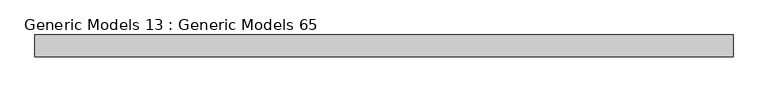
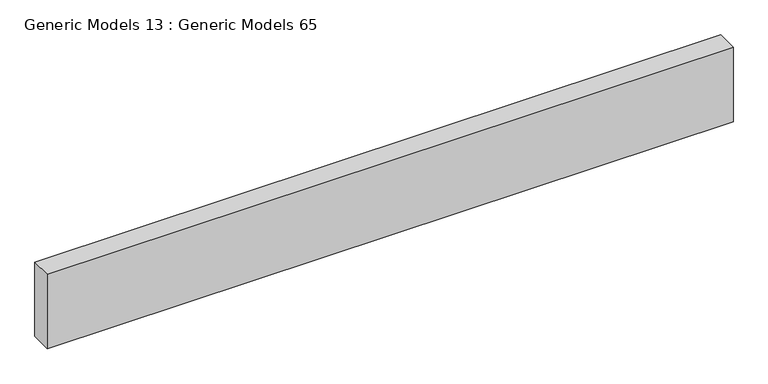
"""IFC4 building model written with IfcOpenShell, lengths in millimetres: proxy geometry, Generic Models 13 : Generic Models 65."""

import ifcopenshell
import ifcopenshell.guid

model = None  # the IFC model being written
_history = None  # IfcOwnerHistory: only IFC2X3 demands one
_inside = {}  # id of a spatial element -> (the spatial element, [elements in it])
_under = {}  # id of a project, library or spatial element -> (it, [spatial elements below it])
_declared = {}  # id of a project -> (the project, [libraries it declares])
_typed = {}  # id of a type object -> (the type object, [elements of that type])
_made_of = {}  # id of a material, layer set ... -> (it, [elements and type objects made of it])


def new_model(schema):
    """Start an empty IFC model of exactly this schema.

    Asked for "IFC4X3", IfcOpenShell would pick the latest addendum, in which some entities
    have other attributes; the version numbers below select the first issue.
    IFC2X3 requires an IfcOwnerHistory on every rooted entity: one is made here for all.
    """
    global model, _history
    if schema == "IFC4X3":
        model = ifcopenshell.file(schema_version=(4, 3, 0, 0))
    else:
        model = ifcopenshell.file(schema=schema)
    _inside.clear()
    _under.clear()
    _declared.clear()
    _typed.clear()
    _made_of.clear()
    _history = None
    if model.schema == "IFC2X3":
        org = make("IfcOrganization", Name="unknown")
        user = make(
            "IfcPersonAndOrganization",
            ThePerson=make("IfcPerson", FamilyName="unknown"),
            TheOrganization=org,
        )
        app = make(
            "IfcApplication",
            ApplicationDeveloper=org,
            Version="unknown",
            ApplicationFullName="unknown",
            ApplicationIdentifier="unknown",
        )
        _history = make(
            "IfcOwnerHistory",
            OwningUser=user,
            OwningApplication=app,
            ChangeAction="ADDED",
            CreationDate=0,
        )
    return model


def make(cls, **values):
    """One entity of the class cls with the attributes given. An attribute that is None is left unset."""
    return model.create_entity(
        cls, **{name: value for name, value in values.items() if value is not None}
    )


def rooted(cls, **values):
    """An entity with a GlobalId (a new one), such as an element, a storey or a relation."""
    return make(cls, GlobalId=ifcopenshell.guid.new(), OwnerHistory=_history, **values)


def si_unit(unit_type, name, prefix=None):
    """IfcSIUnit, for example si_unit("LENGTHUNIT", "METRE", prefix="MILLI")."""
    return make("IfcSIUnit", UnitType=unit_type, Prefix=prefix, Name=name)


def assignment(units):
    """IfcUnitAssignment: the units of a project."""
    return None if units is None else make("IfcUnitAssignment", Units=units)


def point(xyz):
    """IfcCartesianPoint."""
    return None if xyz is None else make("IfcCartesianPoint", Coordinates=xyz)


def direction(xyz):
    """IfcDirection."""
    return None if xyz is None else make("IfcDirection", DirectionRatios=xyz)


def frame(location, z_axis=None, x_axis=None):
    """IfcAxis2Placement3D, a coordinate frame: its origin and axes. An axis left out is left unset."""
    return make(
        "IfcAxis2Placement3D",
        Location=point(location),
        Axis=direction(z_axis),
        RefDirection=direction(x_axis),
    )


def origin():
    """The frame at (0, 0, 0) with its axes left unset."""
    return frame((0.0, 0.0, 0.0))


def place(relative_to, where):
    """IfcLocalPlacement: puts the frame where relative to a parent placement (None: the world)."""
    return make(
        "IfcLocalPlacement", PlacementRelTo=relative_to, RelativePlacement=where
    )


def context(
    kind, dimensions, precision=None, world=None, true_north=None, identifier=None
):
    """IfcGeometricRepresentationContext, for example the 3D "Model" context."""
    return make(
        "IfcGeometricRepresentationContext",
        ContextIdentifier=identifier,
        ContextType=kind,
        CoordinateSpaceDimension=dimensions,
        Precision=precision,
        WorldCoordinateSystem=world,
        TrueNorth=true_north,
    )


def project(units=None, contexts=None):
    """IfcProject with its units and contexts."""
    return rooted(
        "IfcProject",
        Name="project",
        RepresentationContexts=contexts,
        UnitsInContext=assignment(units),
    )


def spatial(cls, under=None, at=None, **own):
    """A site, building, storey or space (cls), placed at a placement, below another one or the project."""
    s = rooted(cls, ObjectPlacement=at, **own)
    if under is not None:
        _under.setdefault(under.id(), (under, []))[1].append(s)
    return s


def polyline(points):
    """IfcPolyline through the points."""
    return make("IfcPolyline", Points=[point(p) for p in points])


def outline(outer, holes=None, kind="AREA"):
    """IfcArbitraryClosedProfileDef: a profile drawn as a closed curve; with holes, ...WithVoids."""
    if holes is None:
        return make("IfcArbitraryClosedProfileDef", ProfileType=kind, OuterCurve=outer)
    return make(
        "IfcArbitraryProfileDefWithVoids",
        ProfileType=kind,
        OuterCurve=outer,
        InnerCurves=holes,
    )


def extrude(swept, where, along, depth):
    """IfcExtrudedAreaSolid: the profile swept, set in the frame where, extruded along a direction by depth."""
    return make(
        "IfcExtrudedAreaSolid",
        SweptArea=swept,
        Position=where,
        ExtrudedDirection=direction(along),
        Depth=depth,
    )


def shape(context_of_items, identifier, shape_type, items):
    """IfcShapeRepresentation: the items that make up one representation, for example the "Body"."""
    return make(
        "IfcShapeRepresentation",
        ContextOfItems=context_of_items,
        RepresentationIdentifier=identifier,
        RepresentationType=shape_type,
        Items=items,
    )


def source(mapping_origin, context_of_items, identifier, shape_type, items):
    """IfcRepresentationMap: a shape defined once, which mapped items show again and again."""
    return make(
        "IfcRepresentationMap",
        MappingOrigin=mapping_origin,
        MappedRepresentation=shape(context_of_items, identifier, shape_type, items),
    )


def transform(
    local_origin,
    x_axis=None,
    y_axis=None,
    z_axis=None,
    scale=None,
    scale2=None,
    scale3=None,
    uniform=True,
):
    """IfcCartesianTransformationOperator3D, or its non-uniform kind. x_axis, y_axis, z_axis: its Axis1, 2, 3."""
    if uniform:
        return make(
            "IfcCartesianTransformationOperator3D",
            Axis1=direction(x_axis),
            Axis2=direction(y_axis),
            LocalOrigin=point(local_origin),
            Scale=scale,
            Axis3=direction(z_axis),
        )
    return make(
        "IfcCartesianTransformationOperator3DnonUniform",
        Axis1=direction(x_axis),
        Axis2=direction(y_axis),
        LocalOrigin=point(local_origin),
        Scale=scale,
        Axis3=direction(z_axis),
        Scale2=scale2,
        Scale3=scale3,
    )


def mapped(mapping_source, mapping_target):
    """IfcMappedItem: shows the shape of a source again, moved by a transform."""
    return make(
        "IfcMappedItem", MappingSource=mapping_source, MappingTarget=mapping_target
    )


def made_of(thing, what):
    """Note that an element or type object is made of a material, layer set ...; save() writes the relation."""
    if what is not None:
        _made_of.setdefault(what.id(), (what, []))[1].append(thing)
    return thing


def element(
    cls,
    number,
    at=None,
    inside=None,
    cuts=None,
    type_object=None,
    material=None,
    context=None,
    identifier="Body",
    shape_type=None,
    held_by="IfcProductDefinitionShape",
    body=None,
    shapes=None,
    **own,
):
    """One element of the class cls, such as IfcWall. Its Tag is "e" and its number.

    at: its placement. inside: the storey or other place that contains it. cuts: it is an
    opening in that element (IfcRelVoidsElement). A single representation is given by context,
    identifier, shape_type and body (its items); several are given by shapes. held_by: the class
    of the entity that holds the representations. save() writes the other relations.
    """
    e = rooted(cls, Tag="e%d" % number, ObjectPlacement=at, **own)
    if body is not None:
        shapes = [shape(context, identifier, shape_type, body)]
    if shapes is not None:
        e.Representation = make(held_by, Representations=shapes)
    if inside is not None:
        _inside.setdefault(inside.id(), (inside, []))[1].append(e)
    if cuts is not None:
        rooted(
            "IfcRelVoidsElement", RelatingBuildingElement=cuts, RelatedOpeningElement=e
        )
    if type_object is not None:
        _typed.setdefault(type_object.id(), (type_object, []))[1].append(e)
    return made_of(e, material)


def aggregate(whole, parts):
    """IfcRelAggregates: a whole, such as a stair, and the parts it consists of."""
    return rooted("IfcRelAggregates", RelatingObject=whole, RelatedObjects=parts)


def save(model, path):
    """Write the relations noted so far, then the file.

    IfcRelAggregates (storeys below a building ...), IfcRelContainedInSpatialStructure (elements
    in a storey), IfcRelDefinesByType, IfcRelAssociatesMaterial and IfcRelDeclares: one each for
    every whole, place, type object, material and project.
    """
    for whole, parts in _under.values():
        aggregate(whole, parts)
    for where, things in _inside.values():
        rooted(
            "IfcRelContainedInSpatialStructure",
            RelatedElements=things,
            RelatingStructure=where,
        )
    for kind, things in _typed.values():
        rooted("IfcRelDefinesByType", RelatedObjects=things, RelatingType=kind)
    for what, things in _made_of.values():
        rooted("IfcRelAssociatesMaterial", RelatedObjects=things, RelatingMaterial=what)
    for by, libraries in _declared.values():
        rooted("IfcRelDeclares", RelatingContext=by, RelatedDefinitions=libraries)
    model.write(path)


def generic_models_13_generic_models_65_9e643fb9(model_context):
    return source(origin(), model_context, "Body", "SweptSolid", [
        extrude(outline(polyline([(49128.3625, 592.1375), (49128.3625, 630.2375), (50347.5625, 630.2375), (50347.5625, 592.1375), (49128.3625, 592.1375)])), frame((0.0, 0.0, 5507.83125), z_axis=(0.0, 0.0, 1.0), x_axis=(1.0, 0.0, 0.0)), (0.0, 0.0, 1.0), 139.7),
    ])


if __name__ == "__main__":
    model = new_model("IFC4")
    model_context = context("Model", 3, world=origin())
    ifc_project = project(units=[si_unit("LENGTHUNIT", "METRE", prefix="MILLI")], contexts=[model_context])
    site = spatial("IfcSite", under=ifc_project)
    building = spatial("IfcBuilding", under=site)
    placement = place(None, origin())
    generic_models_13_generic_models_65_shape = generic_models_13_generic_models_65_9e643fb9(model_context)
    element("IfcBuildingElementProxy", 1, Name="Generic Models 13 : Generic Models 65", ObjectType="Generic Models 13 : Generic Models 65", at=placement, inside=building, context=model_context, shape_type="MappedRepresentation", body=[
        mapped(generic_models_13_generic_models_65_shape, transform((0.0, 0.0, 0.0), x_axis=(1.0, 0.0, 0.0), y_axis=(0.0, 1.0, 0.0), z_axis=(0.0, 0.0, 1.0))),
    ])
    save(model, "model.ifc")

# Revit data of these elements
# Element 1 (IfcBuildingElementProxy, "Generic Models 13 : Generic Models 65")
#   Materials on its faces: "WOOD JOIST AS SPECIFIED"
# Materials
#   "WOOD JOIST AS SPECIFIED": class "Wood", colour RGB 234 198 147, transparency 0, Description = "Pinus Echinata", Cost = 0
